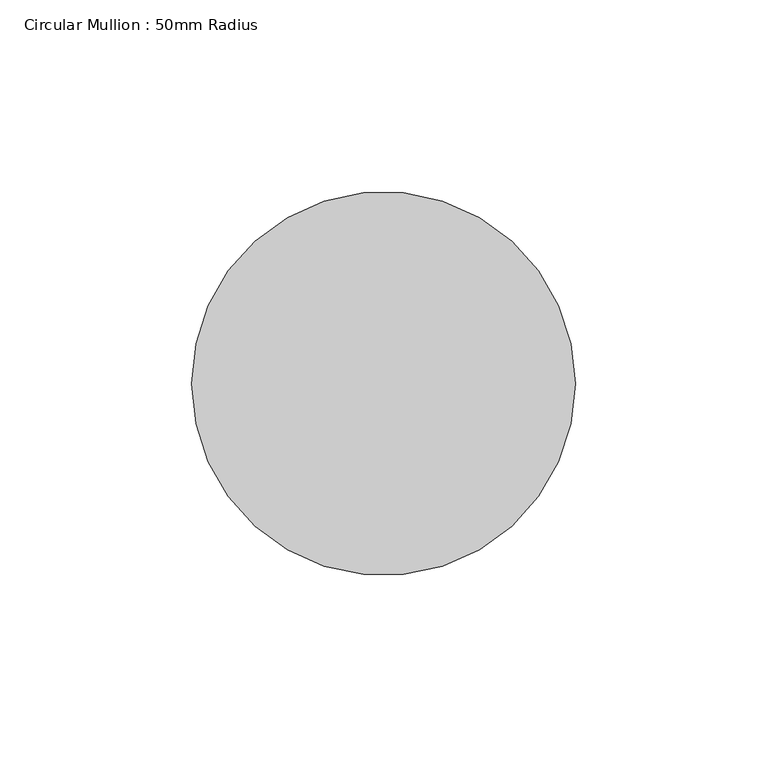
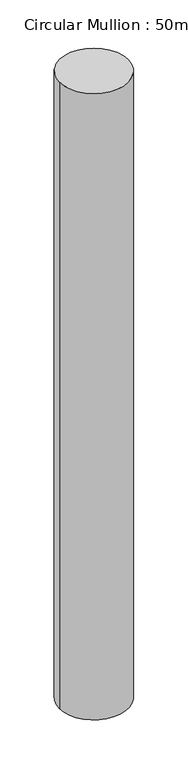
"""IFC4 building model written with IfcOpenShell, lengths in millimetres: member geometry, Circular Mullion : 50mm Radius."""

from ifc_helpers import new_model, si_unit, point, frame, origin, origin_2d, place, context, project, spatial, circle_curve, trimmed, segment, composite_curve, outline, extrude, source, transform, mapped, element, save


def circular_mullion_50mm_radius_f3c4ae2c(model_context):
    return source(origin(), model_context, "Body", "SweptSolid", [
        extrude(outline(composite_curve([segment(trimmed(circle_curve(origin_2d(), 50.0), [point((50.0, 0.0))], [point((-50.0, 0.0))], False, "CARTESIAN"), True, "CONTINUOUS"), segment(trimmed(circle_curve(origin_2d(), 50.0), [point((-50.0, 0.0))], [point((50.0, 0.0))], False, "CARTESIAN"), True, "CONTINUOUS")], self_intersect=False)), frame((0.0, 0.0, -961.7251563), z_axis=(0.0, 0.0, 1.0), x_axis=(1.0, 0.0, 0.0)), (0.0, 0.0, 1.0), 961.7251563),
    ])


if __name__ == "__main__":
    model = new_model("IFC4")
    model_context = context("Model", 3, world=origin())
    ifc_project = project(units=[si_unit("LENGTHUNIT", "METRE", prefix="MILLI")], contexts=[model_context])
    site = spatial("IfcSite", under=ifc_project)
    building = spatial("IfcBuilding", under=site)
    placement = place(None, origin())
    circular_mullion_50mm_radius_shape = circular_mullion_50mm_radius_f3c4ae2c(model_context)
    element("IfcMember", 1, ObjectType="Circular Mullion : 50mm Radius", at=placement, inside=building, context=model_context, shape_type="MappedRepresentation", body=[
        mapped(circular_mullion_50mm_radius_shape, transform((0.0, 0.0, 0.0), x_axis=(1.0, 0.0, 0.0), y_axis=(0.0, 1.0, 0.0), z_axis=(0.0, 0.0, 1.0))),
    ])
    save(model, "model.ifc")

# Revit data of these elements
# Type "Circular Mullion : 50mm Radius"
#   built-in parameter 1007350 = 0.164042 (stored number, unit not read)
# Element 1 (IfcMember, "Circular Mullion : 50mm Radius")
#   Materials on its faces: "Aluminium"
# Materials
#   "Aluminium": class "Metal", colour RGB 247 247 247, transparency 0, Description = "Aluminium 6061", Cost = 0
